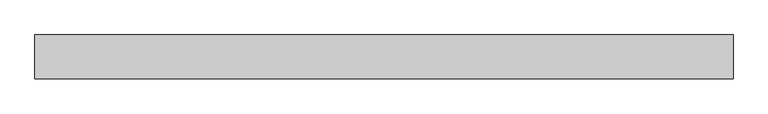
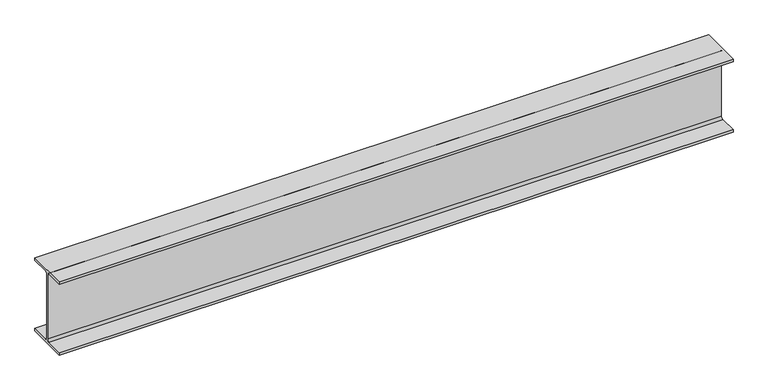
"""IFC4 building model written with IfcOpenShell, lengths in millimetres: beam geometry, Old_Steel Beam_H-KSD3502 : H_SB_ASB_H-250×125x6x9."""

from ifc_helpers import new_model, si_unit, point, frame, frame_2d, origin, place, context, project, spatial, polyline, circle_curve, trimmed, segment, composite_curve, outline, extrude, source, transform, mapped, element, save


def beam_60afac87(model_context):
    return source(origin(), model_context, "Body", "SweptSolid", [
        extrude(outline(composite_curve([segment(polyline([(82.5, -141.5), (82.5, -151.7), (-82.5, -151.7), (-82.5, -141.5), (-11.9, -141.5)]), True, "CONTINUOUS"), segment(trimmed(circle_curve(frame_2d((-11.9, -132.6)), 8.9), [point((-11.9, -141.5))], [point((-3.0, -132.6))], True, "CARTESIAN"), True, "CONTINUOUS"), segment(polyline([(-3.0, -132.6), (-3.0, 132.6)]), True, "CONTINUOUS"), segment(trimmed(circle_curve(frame_2d((-11.9, 132.6)), 8.9), [point((-3.0, 132.6))], [point((-11.9, 141.5))], True, "CARTESIAN"), True, "CONTINUOUS"), segment(polyline([(-11.9, 141.5), (-82.5, 141.5), (-82.5, 151.7), (82.5, 151.7), (82.5, 141.5), (11.9, 141.5)]), True, "CONTINUOUS"), segment(trimmed(circle_curve(frame_2d((11.9, 132.6)), 8.9), [point((11.9, 141.5))], [point((3.0, 132.6))], True, "CARTESIAN"), True, "CONTINUOUS"), segment(polyline([(3.0, 132.6), (3.0, -132.6)]), True, "CONTINUOUS"), segment(trimmed(circle_curve(frame_2d((11.9, -132.6)), 8.9), [point((3.0, -132.6))], [point((11.9, -141.5))], True, "CARTESIAN"), True, "CONTINUOUS"), segment(polyline([(11.9, -141.5), (82.5, -141.5)]), True, "CONTINUOUS")], self_intersect=False)), frame((-1249.3, 0.0, 0.0), z_axis=(1.0, 0.0, 0.0), x_axis=(0.0, 1.0, 0.0)), (0.0, 0.0, 1.0), 2636.6),
    ])


if __name__ == "__main__":
    model = new_model("IFC4")
    model_context = context("Model", 3, world=origin())
    ifc_project = project(units=[si_unit("LENGTHUNIT", "METRE", prefix="MILLI")], contexts=[model_context])
    site = spatial("IfcSite", under=ifc_project)
    building = spatial("IfcBuilding", under=site)
    placement = place(None, origin())
    beam_shape = beam_60afac87(model_context)
    element("IfcBeam", 1, ObjectType="Old_Steel Beam_H-KSD3502 : H_SB_ASB_H-250×125x6x9", at=placement, inside=building, context=model_context, shape_type="MappedRepresentation", body=[
        mapped(beam_shape, transform((0.0, 0.0, 0.0), x_axis=(1.0, 0.0, 0.0), y_axis=(0.0, 1.0, 0.0), z_axis=(0.0, 0.0, 1.0))),
    ])
    save(model, "model.ifc")

# Revit data of these elements
# Type "Old_Steel Beam_H-KSD3502 : H_SB_ASB_H-250×125x6x9"
#   Width = 12.5 cm
#   Web Thickness = 0.6 cm
#   Web Fillet = 1.2 cm
#   Warping Constant = 42539.8 cm⁶
#   Torsional Moment of Inertia = 7.8102 cm⁴
#   Torsional Modulus = 1.0 cm³
#   Section Area = 37.66 cm²
#   Plastic Modulus weak axis = 73.1 cm³
#   Plastic Modulus strong axis = 366.0 cm³
#   Perimeter = 0.97 m²/m
#   Nominal Weight = 29.60 kgf/m
#   Moment of Inertia weak axis = 294.00 cm⁴
#   Moment of Inertia strong axis = 4050.00 cm⁴
#   Height = 25.0 cm
#   Flange Thickness = 0.9 cm
#   Elastic Modulus weak axis = 47.0 cm³
#   Elastic Modulus strong axis = 324.0 cm³
#   Centroid Vertical = 12.5 cm
#   Centroid Horizontal = 6.25 cm
#   Length [instance default] = 1.5240 m
#   Structural Material [instance default] = Steel, 45-345
#   Assembly Code = ""
# Element 1 (IfcBeam, "Old_Steel Beam_H-KSD3502 : H_SB_ASB_H-250×125x6x9")
#   Structural Material = none
# Materials
#   "Steel, 45-345": class "Metal", colour RGB 189 187 185, transparency 0, Description = "Steel 345 MPa", Cost = 0
